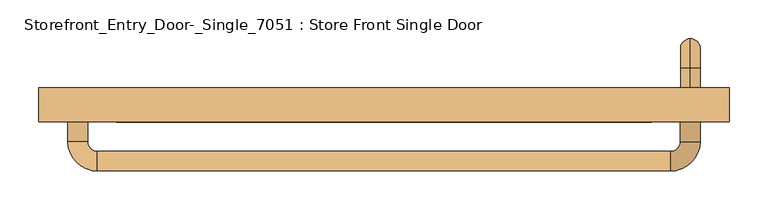
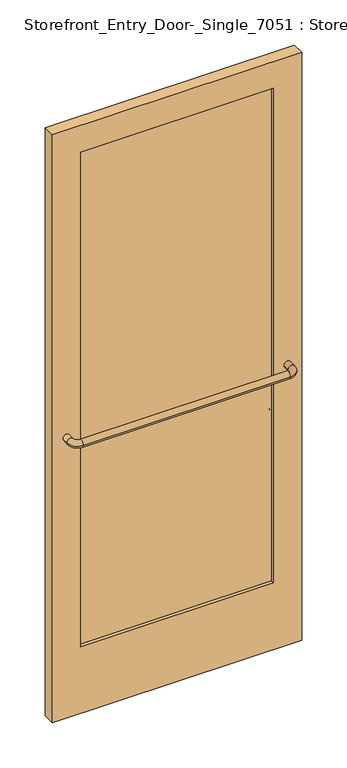
"""IFC4 building model written with IfcOpenShell, lengths in millimetres: door geometry, Storefront_Entry_Door-_Single_7051 : Store Front Single Door."""

import ifcopenshell
import ifcopenshell.guid

model = None  # the IFC model being written
_history = None  # IfcOwnerHistory: only IFC2X3 demands one
_inside = {}  # id of a spatial element -> (the spatial element, [elements in it])
_under = {}  # id of a project, library or spatial element -> (it, [spatial elements below it])
_declared = {}  # id of a project -> (the project, [libraries it declares])
_typed = {}  # id of a type object -> (the type object, [elements of that type])
_made_of = {}  # id of a material, layer set ... -> (it, [elements and type objects made of it])


def new_model(schema):
    """Start an empty IFC model of exactly this schema.

    Asked for "IFC4X3", IfcOpenShell would pick the latest addendum, in which some entities
    have other attributes; the version numbers below select the first issue.
    IFC2X3 requires an IfcOwnerHistory on every rooted entity: one is made here for all.
    """
    global model, _history
    if schema == "IFC4X3":
        model = ifcopenshell.file(schema_version=(4, 3, 0, 0))
    else:
        model = ifcopenshell.file(schema=schema)
    _inside.clear()
    _under.clear()
    _declared.clear()
    _typed.clear()
    _made_of.clear()
    _history = None
    if model.schema == "IFC2X3":
        org = make("IfcOrganization", Name="unknown")
        user = make(
            "IfcPersonAndOrganization",
            ThePerson=make("IfcPerson", FamilyName="unknown"),
            TheOrganization=org,
        )
        app = make(
            "IfcApplication",
            ApplicationDeveloper=org,
            Version="unknown",
            ApplicationFullName="unknown",
            ApplicationIdentifier="unknown",
        )
        _history = make(
            "IfcOwnerHistory",
            OwningUser=user,
            OwningApplication=app,
            ChangeAction="ADDED",
            CreationDate=0,
        )
    return model


def make(cls, **values):
    """One entity of the class cls with the attributes given. An attribute that is None is left unset."""
    return model.create_entity(
        cls, **{name: value for name, value in values.items() if value is not None}
    )


def rooted(cls, **values):
    """An entity with a GlobalId (a new one), such as an element, a storey or a relation."""
    return make(cls, GlobalId=ifcopenshell.guid.new(), OwnerHistory=_history, **values)


def si_unit(unit_type, name, prefix=None):
    """IfcSIUnit, for example si_unit("LENGTHUNIT", "METRE", prefix="MILLI")."""
    return make("IfcSIUnit", UnitType=unit_type, Prefix=prefix, Name=name)


def assignment(units):
    """IfcUnitAssignment: the units of a project."""
    return None if units is None else make("IfcUnitAssignment", Units=units)


def point(xyz):
    """IfcCartesianPoint."""
    return None if xyz is None else make("IfcCartesianPoint", Coordinates=xyz)


def direction(xyz):
    """IfcDirection."""
    return None if xyz is None else make("IfcDirection", DirectionRatios=xyz)


def frame(location, z_axis=None, x_axis=None):
    """IfcAxis2Placement3D, a coordinate frame: its origin and axes. An axis left out is left unset."""
    return make(
        "IfcAxis2Placement3D",
        Location=point(location),
        Axis=direction(z_axis),
        RefDirection=direction(x_axis),
    )


def origin():
    """The frame at (0, 0, 0) with its axes left unset."""
    return frame((0.0, 0.0, 0.0))


def place(relative_to, where):
    """IfcLocalPlacement: puts the frame where relative to a parent placement (None: the world)."""
    return make(
        "IfcLocalPlacement", PlacementRelTo=relative_to, RelativePlacement=where
    )


def context(
    kind, dimensions, precision=None, world=None, true_north=None, identifier=None
):
    """IfcGeometricRepresentationContext, for example the 3D "Model" context."""
    return make(
        "IfcGeometricRepresentationContext",
        ContextIdentifier=identifier,
        ContextType=kind,
        CoordinateSpaceDimension=dimensions,
        Precision=precision,
        WorldCoordinateSystem=world,
        TrueNorth=true_north,
    )


def project(units=None, contexts=None):
    """IfcProject with its units and contexts."""
    return rooted(
        "IfcProject",
        Name="project",
        RepresentationContexts=contexts,
        UnitsInContext=assignment(units),
    )


def spatial(cls, under=None, at=None, **own):
    """A site, building, storey or space (cls), placed at a placement, below another one or the project."""
    s = rooted(cls, ObjectPlacement=at, **own)
    if under is not None:
        _under.setdefault(under.id(), (under, []))[1].append(s)
    return s


def polyline(points):
    """IfcPolyline through the points."""
    return make("IfcPolyline", Points=[point(p) for p in points])


def circle_curve(where, radius):
    """IfcCircle in the frame where."""
    return make("IfcCircle", Position=where, Radius=radius)


def ellipse_curve(where, semi_axis1, semi_axis2):
    """IfcEllipse in the frame where."""
    return make(
        "IfcEllipse", Position=where, SemiAxis1=semi_axis1, SemiAxis2=semi_axis2
    )


def trimmed(basis, trim1, trim2, sense, master):
    """IfcTrimmedCurve: the piece of a basis curve between two trims."""
    return make(
        "IfcTrimmedCurve",
        BasisCurve=basis,
        Trim1=trim1,
        Trim2=trim2,
        SenseAgreement=sense,
        MasterRepresentation=master,
    )


def outline(outer, holes=None, kind="AREA"):
    """IfcArbitraryClosedProfileDef: a profile drawn as a closed curve; with holes, ...WithVoids."""
    if holes is None:
        return make("IfcArbitraryClosedProfileDef", ProfileType=kind, OuterCurve=outer)
    return make(
        "IfcArbitraryProfileDefWithVoids",
        ProfileType=kind,
        OuterCurve=outer,
        InnerCurves=holes,
    )


def extrude(swept, where, along, depth):
    """IfcExtrudedAreaSolid: the profile swept, set in the frame where, extruded along a direction by depth."""
    return make(
        "IfcExtrudedAreaSolid",
        SweptArea=swept,
        Position=where,
        ExtrudedDirection=direction(along),
        Depth=depth,
    )


def shape(context_of_items, identifier, shape_type, items):
    """IfcShapeRepresentation: the items that make up one representation, for example the "Body"."""
    return make(
        "IfcShapeRepresentation",
        ContextOfItems=context_of_items,
        RepresentationIdentifier=identifier,
        RepresentationType=shape_type,
        Items=items,
    )


def source(mapping_origin, context_of_items, identifier, shape_type, items):
    """IfcRepresentationMap: a shape defined once, which mapped items show again and again."""
    return make(
        "IfcRepresentationMap",
        MappingOrigin=mapping_origin,
        MappedRepresentation=shape(context_of_items, identifier, shape_type, items),
    )


def transform(
    local_origin,
    x_axis=None,
    y_axis=None,
    z_axis=None,
    scale=None,
    scale2=None,
    scale3=None,
    uniform=True,
):
    """IfcCartesianTransformationOperator3D, or its non-uniform kind. x_axis, y_axis, z_axis: its Axis1, 2, 3."""
    if uniform:
        return make(
            "IfcCartesianTransformationOperator3D",
            Axis1=direction(x_axis),
            Axis2=direction(y_axis),
            LocalOrigin=point(local_origin),
            Scale=scale,
            Axis3=direction(z_axis),
        )
    return make(
        "IfcCartesianTransformationOperator3DnonUniform",
        Axis1=direction(x_axis),
        Axis2=direction(y_axis),
        LocalOrigin=point(local_origin),
        Scale=scale,
        Axis3=direction(z_axis),
        Scale2=scale2,
        Scale3=scale3,
    )


def mapped(mapping_source, mapping_target):
    """IfcMappedItem: shows the shape of a source again, moved by a transform."""
    return make(
        "IfcMappedItem", MappingSource=mapping_source, MappingTarget=mapping_target
    )


def made_of(thing, what):
    """Note that an element or type object is made of a material, layer set ...; save() writes the relation."""
    if what is not None:
        _made_of.setdefault(what.id(), (what, []))[1].append(thing)
    return thing


def element(
    cls,
    number,
    at=None,
    inside=None,
    cuts=None,
    type_object=None,
    material=None,
    context=None,
    identifier="Body",
    shape_type=None,
    held_by="IfcProductDefinitionShape",
    body=None,
    shapes=None,
    **own,
):
    """One element of the class cls, such as IfcWall. Its Tag is "e" and its number.

    at: its placement. inside: the storey or other place that contains it. cuts: it is an
    opening in that element (IfcRelVoidsElement). A single representation is given by context,
    identifier, shape_type and body (its items); several are given by shapes. held_by: the class
    of the entity that holds the representations. save() writes the other relations.
    """
    e = rooted(cls, Tag="e%d" % number, ObjectPlacement=at, **own)
    if body is not None:
        shapes = [shape(context, identifier, shape_type, body)]
    if shapes is not None:
        e.Representation = make(held_by, Representations=shapes)
    if inside is not None:
        _inside.setdefault(inside.id(), (inside, []))[1].append(e)
    if cuts is not None:
        rooted(
            "IfcRelVoidsElement", RelatingBuildingElement=cuts, RelatedOpeningElement=e
        )
    if type_object is not None:
        _typed.setdefault(type_object.id(), (type_object, []))[1].append(e)
    return made_of(e, material)


def aggregate(whole, parts):
    """IfcRelAggregates: a whole, such as a stair, and the parts it consists of."""
    return rooted("IfcRelAggregates", RelatingObject=whole, RelatedObjects=parts)


def save(model, path):
    """Write the relations noted so far, then the file.

    IfcRelAggregates (storeys below a building ...), IfcRelContainedInSpatialStructure (elements
    in a storey), IfcRelDefinesByType, IfcRelAssociatesMaterial and IfcRelDeclares: one each for
    every whole, place, type object, material and project.
    """
    for whole, parts in _under.values():
        aggregate(whole, parts)
    for where, things in _inside.values():
        rooted(
            "IfcRelContainedInSpatialStructure",
            RelatedElements=things,
            RelatingStructure=where,
        )
    for kind, things in _typed.values():
        rooted("IfcRelDefinesByType", RelatedObjects=things, RelatingType=kind)
    for what, things in _made_of.values():
        rooted("IfcRelAssociatesMaterial", RelatedObjects=things, RelatingMaterial=what)
    for by, libraries in _declared.values():
        rooted("IfcRelDeclares", RelatingContext=by, RelatedDefinitions=libraries)
    model.write(path)


def plane_surface(at):
    """IfcPlane: the flat surface through the origin of the frame at, square to its z axis."""
    return make("IfcPlane", Position=at)


def cylinder_surface(at, radius):
    """IfcCylindricalSurface: all points at the distance radius from the z axis of the frame at."""
    return make("IfcCylindricalSurface", Position=at, Radius=radius)


def revolved_surface(curve, axis_point, axis_direction):
    """IfcSurfaceOfRevolution: the curve turned about the line through axis_point along axis_direction."""
    return make(
        "IfcSurfaceOfRevolution",
        SweptCurve=make("IfcArbitraryOpenProfileDef", ProfileType="CURVE", Curve=curve),
        AxisPosition=make("IfcAxis1Placement", Location=point(axis_point), Axis=direction(axis_direction)),
    )


def advanced_brep(points, edges, surfaces, faces):
    """IfcAdvancedBrep: a solid bounded by faces that lie on surfaces and meet in shared edges.

    An edge is (start, end): straight between two places in points (the first is 0);
    or (start, end, curve); or (start, end, curve, False) where it runs against its curve.
    A face is (place in surfaces, loops), or (place, loops, False) where it looks against
    its surface's normal. A loop lists edges by number (the first is 1), with a minus sign
    where the edge is run from its end to its start. The first loop is the outer one.
    """
    corners = [point(p) for p in points]
    vertices = [make("IfcVertexPoint", VertexGeometry=c) for c in corners]
    made = []
    for start, end, *more in edges:
        made.append(
            make(
                "IfcEdgeCurve",
                EdgeStart=vertices[start],
                EdgeEnd=vertices[end],
                EdgeGeometry=more[0] if more else make("IfcPolyline", Points=[corners[start], corners[end]]),
                SameSense=more[1] if len(more) > 1 else True,
            )
        )
    hull = []
    for where, loops, *sense in faces:
        bounds = []
        for j, loop in enumerate(loops):
            ring = [make("IfcOrientedEdge", EdgeElement=made[abs(k) - 1], Orientation=k > 0) for k in loop]
            bounds.append(
                make(
                    "IfcFaceOuterBound" if j == 0 else "IfcFaceBound",
                    Bound=make("IfcEdgeLoop", EdgeList=ring),
                    Orientation=True,
                )
            )
        hull.append(make("IfcAdvancedFace", Bounds=bounds, FaceSurface=surfaces[where], SameSense=sense[0] if sense else True))
    return make("IfcAdvancedBrep", Outer=make("IfcClosedShell", CfsFaces=hull))


def storefront_entry_door_single_7051_store_front_single_door_d505028f(model_context):
    return source(origin(), model_context, "Body", "SolidModel", [
        advanced_brep(
        [(397.2894329, 50.8, 1054.1), (397.2894329, 50.8, 1079.5), (397.2894329, 76.2, 1054.1), (397.2894329, 76.2, 1079.5), (397.2894329, 114.3, 1041.4), (397.2894329, 88.9, 1041.4), (397.2894329, 88.9, 863.6), (397.2894329, 114.3, 863.6), (397.2894329, 76.2, 825.5), (397.2894329, 76.2, 850.9), (397.2894329, 50.8, 850.9), (397.2894329, 50.8, 825.5)],
        [
            (0, 1, circle_curve(frame((397.2894329, 50.8, 1066.8), z_axis=(0.0, -1.0, 0.0), x_axis=(0.0, 0.0, 1.0)), 12.7)),
            (1, 0, circle_curve(frame((397.2894329, 50.8, 1066.8), z_axis=(0.0, -1.0, 0.0), x_axis=(0.0, 0.0, 1.0)), 12.7)),
            (0, 2),
            (2, 3, circle_curve(frame((397.2894329, 76.2, 1066.8), z_axis=(0.0, -1.0, 0.0), x_axis=(0.0, 0.0, 1.0)), 12.7)),
            (3, 1),
            (3, 2, circle_curve(frame((397.2894329, 76.2, 1066.8), z_axis=(0.0, -1.0, 0.0), x_axis=(0.0, 0.0, 1.0)), 12.7)),
            (4, 3, circle_curve(frame((397.2894329, 76.2, 1041.4), z_axis=(1.0, 0.0, 0.0), x_axis=(0.0, 0.0, 1.0)), 38.1)),
            (2, 5, circle_curve(frame((397.2894329, 76.2, 1041.4), z_axis=(-1.0, 0.0, 0.0), x_axis=(0.0, 0.0, 1.0)), 12.7)),
            (5, 4, circle_curve(frame((397.2894329, 101.6, 1041.4), z_axis=(0.0, 0.0, 1.0), x_axis=(0.0, 1.0, 0.0)), 12.7)),
            (4, 5, circle_curve(frame((397.2894329, 101.6, 1041.4), z_axis=(0.0, 0.0, 1.0), x_axis=(0.0, 1.0, 0.0)), 12.7)),
            (5, 6),
            (6, 7, circle_curve(frame((397.2894329, 101.6, 863.6), z_axis=(0.0, 0.0, 1.0), x_axis=(0.0, 1.0, 0.0)), 12.7)),
            (7, 4),
            (7, 6, circle_curve(frame((397.2894329, 101.6, 863.6), z_axis=(0.0, 0.0, 1.0), x_axis=(0.0, 1.0, 0.0)), 12.7)),
            (8, 7, circle_curve(frame((397.2894329, 76.2, 863.6), z_axis=(1.0, 0.0, 0.0), x_axis=(0.0, 1.0, 0.0)), 38.1)),
            (6, 9, circle_curve(frame((397.2894329, 76.2, 863.6), z_axis=(-1.0, 0.0, 0.0), x_axis=(0.0, 1.0, 0.0)), 12.7)),
            (9, 8, circle_curve(frame((397.2894329, 76.2, 838.2), z_axis=(0.0, 1.0, 0.0), x_axis=(0.0, 0.0, -1.0)), 12.7)),
            (8, 9, circle_curve(frame((397.2894329, 76.2, 838.2), z_axis=(0.0, 1.0, 0.0), x_axis=(0.0, 0.0, -1.0)), 12.7)),
            (10, 11, circle_curve(frame((397.2894329, 50.8, 838.2), z_axis=(0.0, -1.0, 0.0), x_axis=(0.0, 0.0, -1.0)), 12.7)),
            (11, 10, circle_curve(frame((397.2894329, 50.8, 838.2), z_axis=(0.0, -1.0, 0.0), x_axis=(0.0, 0.0, -1.0)), 12.7)),
            (9, 10),
            (11, 8),
        ],
        [
            plane_surface(frame((397.2894329, 50.8, 1066.8), z_axis=(0.0, -1.0, 0.0), x_axis=(1.0, 0.0, 0.0))),
            cylinder_surface(frame((397.2894329, 50.8, 1066.8), z_axis=(0.0, -1.0, 0.0), x_axis=(0.0, 0.0, 1.0)), 12.7),
            revolved_surface(trimmed(ellipse_curve(frame((397.2894329, 76.2, 1066.8), z_axis=(0.0, -1.0, 0.0), x_axis=(0.0, 0.0, 1.0)), 12.7, 12.7), [point((397.2894329, 76.2, 1054.1))], [point((397.2894329, 76.2, 1079.5))], True, "CARTESIAN"), (397.2894329, 76.2, 1041.4), (-1.0, 0.0, 0.0)),
            revolved_surface(trimmed(ellipse_curve(frame((397.2894329, 76.2, 1066.8), z_axis=(0.0, -1.0, 0.0), x_axis=(0.0, 0.0, 1.0)), 12.7, 12.7), [point((397.2894329, 76.2, 1079.5))], [point((397.2894329, 76.2, 1054.1))], True, "CARTESIAN"), (397.2894329, 76.2, 1041.4), (-1.0, 0.0, 0.0)),
            cylinder_surface(frame((397.2894329, 101.6, 1041.4), z_axis=(0.0, 0.0, 1.0), x_axis=(0.0, 1.0, 0.0)), 12.7),
            revolved_surface(trimmed(ellipse_curve(frame((397.2894329, 101.6, 863.6), z_axis=(0.0, 0.0, 1.0), x_axis=(0.0, 1.0, 0.0)), 12.7, 12.7), [point((397.2894329, 88.9, 863.6))], [point((397.2894329, 114.3, 863.6))], True, "CARTESIAN"), (397.2894329, 76.2, 863.6), (-1.0, 0.0, 0.0)),
            revolved_surface(trimmed(ellipse_curve(frame((397.2894329, 101.6, 863.6), z_axis=(0.0, 0.0, 1.0), x_axis=(0.0, 1.0, 0.0)), 12.7, 12.7), [point((397.2894329, 114.3, 863.6))], [point((397.2894329, 88.9, 863.6))], True, "CARTESIAN"), (397.2894329, 76.2, 863.6), (-1.0, 0.0, 0.0)),
            plane_surface(frame((397.2894329, 50.8, 838.2), z_axis=(0.0, -1.0, 0.0), x_axis=(1.0, 0.0, 0.0))),
            cylinder_surface(frame((397.2894329, 76.2, 838.2), z_axis=(0.0, 1.0, 0.0), x_axis=(0.0, 0.0, -1.0)), 12.7),
        ],
        [
            (0, [[1, 2]]),
            (1, [[-1, 3, 4, 5]]),
            (1, [[-2, -5, 6, -3]]),
            (2, [[7, -4, 8, 9]]),
            (3, [[-8, -6, -7, 10]]),
            (4, [[-9, 11, 12, 13]]),
            (4, [[-10, -13, 14, -11]]),
            (5, [[15, -12, 16, 17]]),
            (6, [[-16, -14, -15, 18]]),
            (7, [[19, 20]]),
            (8, [[-17, 21, -20, 22]]),
            (8, [[-18, -22, -19, -21]]),
        ],
    ),
        advanced_brep(
        [(384.5894329, 6.35, 1066.8), (409.9894329, 6.35, 1066.8), (384.5894329, -19.05, 1066.8), (409.9894329, -19.05, 1066.8), (371.8894329, -57.15, 1066.8), (371.8894329, -31.75, 1066.8), (-371.8894329, -31.75, 1066.8), (-371.8894329, -57.15, 1066.8), (-409.9894329, -19.05, 1066.8), (-384.5894329, -19.05, 1066.8), (-384.5894329, 6.35, 1066.8), (-409.9894329, 6.35, 1066.8)],
        [
            (0, 1, circle_curve(frame((397.2894329, 6.35, 1066.8), z_axis=(0.0, 1.0, 0.0), x_axis=(1.0, 0.0, 0.0)), 12.7)),
            (1, 0, circle_curve(frame((397.2894329, 6.35, 1066.8), z_axis=(0.0, 1.0, 0.0), x_axis=(1.0, 0.0, 0.0)), 12.7)),
            (0, 2),
            (2, 3, circle_curve(frame((397.2894329, -19.05, 1066.8), z_axis=(0.0, 1.0, 0.0), x_axis=(1.0, 0.0, 0.0)), 12.7)),
            (3, 1),
            (3, 2, circle_curve(frame((397.2894329, -19.05, 1066.8), z_axis=(0.0, 1.0, 0.0), x_axis=(1.0, 0.0, 0.0)), 12.7)),
            (4, 3, circle_curve(frame((371.8894329, -19.05, 1066.8), z_axis=(0.0, 0.0, 1.0), x_axis=(1.0, 0.0, 0.0)), 38.1)),
            (2, 5, circle_curve(frame((371.8894329, -19.05, 1066.8), z_axis=(0.0, 0.0, -1.0), x_axis=(1.0, 0.0, 0.0)), 12.7)),
            (5, 4, circle_curve(frame((371.8894329, -44.45, 1066.8), z_axis=(1.0, 0.0, 0.0), x_axis=(0.0, -1.0, 0.0)), 12.7)),
            (4, 5, circle_curve(frame((371.8894329, -44.45, 1066.8), z_axis=(1.0, 0.0, 0.0), x_axis=(0.0, -1.0, 0.0)), 12.7)),
            (5, 6),
            (6, 7, circle_curve(frame((-371.8894329, -44.45, 1066.8), z_axis=(1.0, 0.0, 0.0), x_axis=(0.0, -1.0, 0.0)), 12.7)),
            (7, 4),
            (7, 6, circle_curve(frame((-371.8894329, -44.45, 1066.8), z_axis=(1.0, 0.0, 0.0), x_axis=(0.0, -1.0, 0.0)), 12.7)),
            (8, 7, circle_curve(frame((-371.8894329, -19.05, 1066.8), z_axis=(0.0, 0.0, 1.0), x_axis=(0.0, -1.0, 0.0)), 38.1)),
            (6, 9, circle_curve(frame((-371.8894329, -19.05, 1066.8), z_axis=(0.0, 0.0, -1.0), x_axis=(0.0, -1.0, 0.0)), 12.7)),
            (9, 8, circle_curve(frame((-397.2894329, -19.05, 1066.8), z_axis=(0.0, -1.0, 0.0), x_axis=(-1.0, 0.0, 0.0)), 12.7)),
            (8, 9, circle_curve(frame((-397.2894329, -19.05, 1066.8), z_axis=(0.0, -1.0, 0.0), x_axis=(-1.0, 0.0, 0.0)), 12.7)),
            (10, 11, circle_curve(frame((-397.2894329, 6.35, 1066.8), z_axis=(0.0, 1.0, 0.0), x_axis=(-1.0, 0.0, 0.0)), 12.7)),
            (11, 10, circle_curve(frame((-397.2894329, 6.35, 1066.8), z_axis=(0.0, 1.0, 0.0), x_axis=(-1.0, 0.0, 0.0)), 12.7)),
            (9, 10),
            (11, 8),
        ],
        [
            plane_surface(frame((397.2894329, 6.35, 1066.8), z_axis=(0.0, 1.0, 0.0), x_axis=(0.0, 0.0, 1.0))),
            cylinder_surface(frame((397.2894329, 6.35, 1066.8), z_axis=(0.0, 1.0, 0.0), x_axis=(1.0, 0.0, 0.0)), 12.7),
            revolved_surface(trimmed(ellipse_curve(frame((397.2894329, -19.05, 1066.8), z_axis=(0.0, 1.0, 0.0), x_axis=(1.0, 0.0, 0.0)), 12.7, 12.7), [point((384.5894329, -19.05, 1066.8))], [point((409.9894329, -19.05, 1066.8))], True, "CARTESIAN"), (371.8894329, -19.05, 1066.8), (0.0, 0.0, -1.0)),
            revolved_surface(trimmed(ellipse_curve(frame((397.2894329, -19.05, 1066.8), z_axis=(0.0, 1.0, 0.0), x_axis=(1.0, 0.0, 0.0)), 12.7, 12.7), [point((409.9894329, -19.05, 1066.8))], [point((384.5894329, -19.05, 1066.8))], True, "CARTESIAN"), (371.8894329, -19.05, 1066.8), (0.0, 0.0, -1.0)),
            cylinder_surface(frame((371.8894329, -44.45, 1066.8), z_axis=(1.0, 0.0, 0.0), x_axis=(0.0, -1.0, 0.0)), 12.7),
            revolved_surface(trimmed(ellipse_curve(frame((-371.8894329, -44.45, 1066.8), z_axis=(1.0, 0.0, 0.0), x_axis=(0.0, -1.0, 0.0)), 12.7, 12.7), [point((-371.8894329, -31.75, 1066.8))], [point((-371.8894329, -57.15, 1066.8))], True, "CARTESIAN"), (-371.8894329, -19.05, 1066.8), (0.0, 0.0, -1.0)),
            revolved_surface(trimmed(ellipse_curve(frame((-371.8894329, -44.45, 1066.8), z_axis=(1.0, 0.0, 0.0), x_axis=(0.0, -1.0, 0.0)), 12.7, 12.7), [point((-371.8894329, -57.15, 1066.8))], [point((-371.8894329, -31.75, 1066.8))], True, "CARTESIAN"), (-371.8894329, -19.05, 1066.8), (0.0, 0.0, -1.0)),
            plane_surface(frame((-397.2894329, 6.35, 1066.8), z_axis=(0.0, 1.0, 0.0), x_axis=(0.0, 0.0, 1.0))),
            cylinder_surface(frame((-397.2894329, -19.05, 1066.8), z_axis=(0.0, -1.0, 0.0), x_axis=(-1.0, 0.0, 0.0)), 12.7),
        ],
        [
            (0, [[1, 2]]),
            (1, [[-1, 3, 4, 5]]),
            (1, [[-2, -5, 6, -3]]),
            (2, [[7, -4, 8, 9]]),
            (3, [[-8, -6, -7, 10]]),
            (4, [[-9, 11, 12, 13]]),
            (4, [[-10, -13, 14, -11]]),
            (5, [[15, -12, 16, 17]]),
            (6, [[-16, -14, -15, 18]]),
            (7, [[19, 20]]),
            (8, [[-17, 21, -20, 22]]),
            (8, [[-18, -22, -19, -21]]),
        ],
    ),
        extrude(outline(polyline([(346.4894329, 19.05), (-346.4894329, 19.05), (-346.4894329, 38.1), (346.4894329, 38.1), (346.4894329, 19.05)])), frame((0.0, 0.0, 254.0), z_axis=(0.0, 0.0, 1.0), x_axis=(1.0, 0.0, 0.0)), (0.0, 0.0, 1.0), 1879.6),
        extrude(outline(polyline([(2235.2, 448.0894329), (2235.2, -448.0894329), (0.0, -448.0894329), (0.0, 448.0894329), (2235.2, 448.0894329)]), holes=[polyline([(2133.6, -346.4894329), (2133.6, 346.4894329), (254.0, 346.4894329), (254.0, -346.4894329), (2133.6, -346.4894329)])]), frame((0.0, 6.35, 0.0), z_axis=(0.0, 1.0, 0.0), x_axis=(0.0, 0.0, 1.0)), (0.0, 0.0, 1.0), 44.45),
    ])


if __name__ == "__main__":
    model = new_model("IFC4")
    model_context = context("Model", 3, world=origin())
    ifc_project = project(units=[si_unit("LENGTHUNIT", "METRE", prefix="MILLI")], contexts=[model_context])
    site = spatial("IfcSite", under=ifc_project)
    building = spatial("IfcBuilding", under=site)
    placement = place(None, origin())
    storefront_entry_door_single_7051_store_front_single_door_shape = storefront_entry_door_single_7051_store_front_single_door_d505028f(model_context)
    element("IfcDoor", 1, ObjectType="Storefront_Entry_Door-_Single_7051 : Store Front Single Door", at=placement, inside=building, context=model_context, shape_type="MappedRepresentation", body=[
        mapped(storefront_entry_door_single_7051_store_front_single_door_shape, transform((0.0, 0.0, 0.0), x_axis=(1.0, 0.0, 0.0), y_axis=(0.0, 1.0, 0.0), z_axis=(0.0, 0.0, 1.0))),
    ])
    save(model, "model.ifc")

# Revit data of these elements
# Type "Storefront_Entry_Door-_Single_7051 : Store Front Single Door"
#   Type Mark = "19"
#   Assembly Code = "B2030110"
#   Analytic Construction = "<None>"
#   Top Rail = 0' - 4"
#   Side Rail = 0' - 4"
#   Reporting Width [instance default] = 4' - 2"
#   Rail Height AFF = 3' - 6"
#   Offset = 0' - 2"
#   Door Width [instance default] = 4' - 2"
#   Bottom Rail Width = 0' - 10"
#   Material = PAINTED STEEL C CHANNEL
#   Glazing Material = BUTT GLAZED STOREFRONT WITH VERTICAL MULLION
#   Function = (empty or 0)
# Element 1 (IfcDoor, "Storefront_Entry_Door-_Single_7051 : Store Front Single Door")
#   Reporting Width = 2' - 11.28263"
#   Door Width = 2' - 11.28263"
#   Materials on its faces: "PAINTED STEEL C CHANNEL", "BUTT GLAZED STOREFRONT WITH VERTICAL MULLION"
# Materials
#   "PAINTED STEEL C CHANNEL": class "Generic", colour RGB 88 62 61, transparency 0, Cost = 0
#   "BUTT GLAZED STOREFRONT WITH VERTICAL MULLION": class "Glass", colour RGB 236 240 239, transparency 0.39, Description = "Soda Lime Glass", Cost = 0
